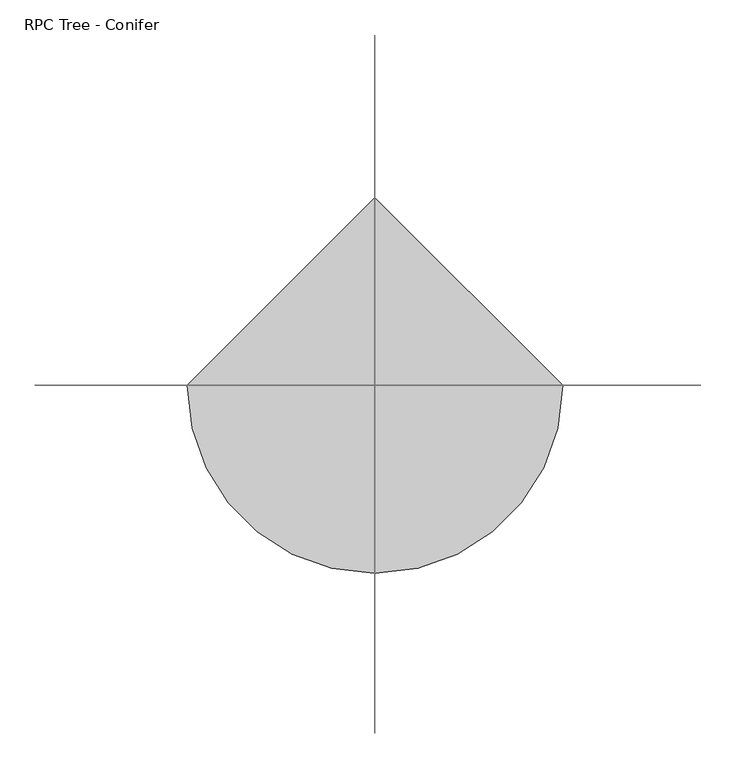
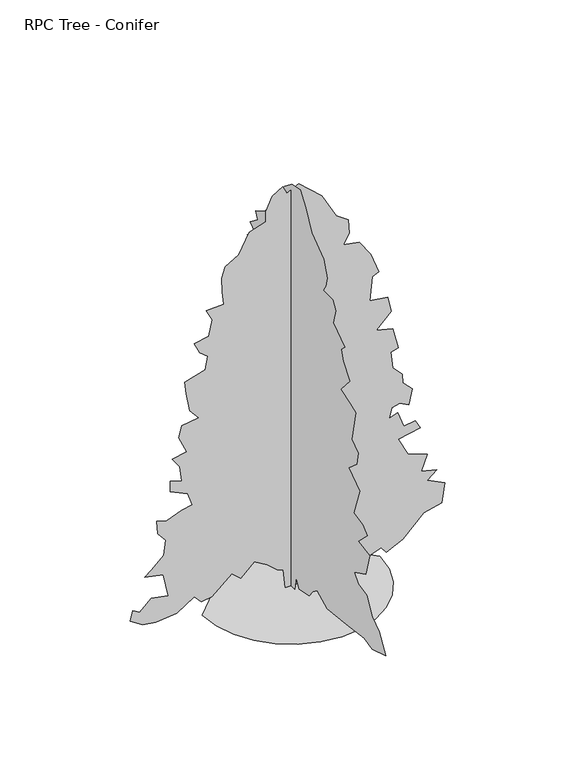
"""IFC4 building model written with IfcOpenShell, lengths in millimetres: geographic element geometry, RPC Tree - Conifer : Colorado Spruce - 4.0 Meters."""

from ifc_helpers import new_model, si_unit, origin, place, context, project, spatial, triangles, source, transform, mapped, element, save


def rpc_tree_conifer_283005fb(model_context):
    return source(origin(), model_context, "Body", "Tessellation", [
        triangles([(0.1966733, 49.8244978, 3.62e-05), (0.1966808, 76.8972503, 209.8139919), (0.1966851, 110.7382534, 304.5674924), (0.1966885, 232.565492, 236.886758), (0.1966934, 381.4650152, 175.9729979), (0.1967001, 550.6699851, 148.90025), (0.1967079, 720.3449844, 156.1022449), (0.1967054, 740.1799656, 40.6092491), (0.1967132, 862.0074858, 121.827502), (0.1967165, 991.2750315, 36.3350005), (0.1967216, 1085.3575155, 67.6820016), (0.1967296, 1268.1000675, 60.913751), (0.1967359, 1356.0849586, 142.1320039), (0.1967499, 1545.5950481, 324.872503), (0.1967463, 1430.5350655, 379.0174902), (0.1967428, 1329.0124832, 412.8600102), (0.1967383, 1234.4449997, 404.9599837), (0.1967407, 1213.9525005, 514.3824835), (0.1967447, 1241.024976, 609.1374919), (0.1967522, 1335.779948, 717.4275026), (0.1967485, 1241.024976, 737.7325132), (0.1967539, 1315.4749374, 805.4150099), (0.1967498, 1200.4174982, 839.2550228), (0.1967461, 1078.589978, 900.169982), (0.1967471, 1015.9549931, 1025.5049915), (0.1967554, 1173.3450228, 1069.3749882), (0.1967602, 1241.024976, 1130.2874765), (0.1967569, 1153.0400122, 1150.5924871), (0.1967529, 1004.1400166, 1238.5800671), (0.1967593, 1112.429991, 1292.7250179), (0.196765, 1121.189994, 1470.9574528), (0.19676, 997.3700083, 1489.0025723), (0.196756, 889.0800339, 1516.0750477), (0.1967604, 905.0550035, 1639.3949913), (0.1967674, 1036.9399767, 1676.5725185), (0.1967726, 1065.0525049, 1807.1074287), (0.1967671, 956.7625305, 1786.8025635), (0.196768, 888.3749897, 1918.5275173), (0.1967741, 963.5299953, 2010.1524479), (0.1967722, 868.7750233, 2091.3700195), (0.1967785, 963.5299953, 2159.0525162), (0.1967813, 990.6024708, 2213.197467), (0.196777, 821.3974646, 2321.4899849), (0.1967781, 801.0925266, 2389.1700108), (0.1967862, 936.4575199, 2456.8523621), (0.1967861, 875.5424881, 2544.8498978), (0.1967818, 740.1799656, 2605.7499596), (0.1967888, 828.1650021, 2707.2748672), (0.1967872, 733.41003, 2795.2500206), (0.1967844, 611.5849806, 2883.2498817), (0.1967873, 604.8150086, 2991.5499573), (0.1967932, 706.3374819, 3038.9249725), (0.1967915, 631.8899912, 3093.074865), (0.1967882, 543.9024839, 3113.3750793), (0.1967957, 658.9624666, 3194.5750648), (0.1967931, 537.1349828, 3289.3500938), (0.1967966, 570.9749957, 3357.0250328), (0.1967927, 428.8425013, 3438.2500168), (0.1967912, 313.7824822, 3560.0751389), (0.1967925, 237.8634971, 3716.3499023), (0.1967912, 97.2017522, 3884.9500763), (0.196789, -11.0894496, 3972.924939), (0.1967837, -146.4532518, 4000.0000305), (0.1967759, -241.2080059, 3878.1749084), (0.196766, -335.9624874, 3688.6751381), (0.196753, -532.2400054, 3546.5250938), (0.1967459, -586.3849926, 3390.8750015), (0.1967443, -559.3125172, 3296.0999725), (0.196744, -525.4725042, 3235.1999107), (0.1967374, -674.3724998, 3235.1999107), (0.1967328, -721.7499859, 3153.9749268), (0.1967304, -681.1399647, 3011.849881), (0.1967181, -870.6499815, 2883.2498817), (0.1967192, -809.7350224, 2829.0999893), (0.1967147, -843.5775061, 2727.5750816), (0.196706, -951.8674805, 2598.9750824), (0.1967076, -802.9674849, 2429.780032), (0.1966991, -959.7425085, 2380.804969), (0.1966941, -1046.6225252, 2341.7949955), (0.1966879, -985.7074934, 2043.9925335), (0.1966812, -1087.2324738, 1969.542572), (0.1966785, -1066.9275358, 1847.7149792), (0.1966808, -938.3300074, 1732.6574673), (0.1966693, -1114.3050219, 1610.8300198), (0.1966655, -1012.7825123, 1333.3325684), (0.1966581, -1161.6825079, 1306.2599476), (0.1966529, -1236.132542, 1245.3475319), (0.1966552, -1087.2324738, 1096.4475363), (0.1966459, -1276.7399471, 1069.3749882), (0.1966422, -1209.0599939, 846.0224876), (0.1966478, -1026.3175146, 758.0375238), (0.1966426, -1087.2324738, 676.8200249), (0.1966355, -1229.3624611, 649.7474768), (0.1966269, -1317.3499683, 494.0775092), (0.1966194, -1432.409951, 412.8600102), (0.1966096, -1533.9325333, 236.886758), (0.1966172, -1317.3499683, 169.2047519), (0.1966241, -1184.517524, 199.5652534), (0.1966359, -895.4949766, 164.0745054), (0.1966487, -586.3849926, 128.5955028), (0.1966584, -423.9474875, 209.8139919), (0.1966598, -356.267498, 155.6682416), (0.1966603, -295.3525025, 81.2182529), (0.1966665, -132.9167506, 47.3774997), (0.1966712, -85.8942484, 133.3167535), (0.1966685, -58.4667483, 3.3e-05), (-51.204578, 1.3e-06, 3.62e-05), (-71.5090799, -2.08e-05, 182.7412439), (-125.6545758, -2.01e-05, 203.0457458), (-220.4093299, -2.09e-05, 284.2650071), (-342.2358327, -2.06e-05, 358.7149867), (-470.8333248, 3.2e-06, 236.886758), (-552.0508238, 2.3e-06, 311.3375007), (-741.5608406, 1.52e-05, 148.90025), (-836.7233459, 1.86e-05, 136.9905027), (-903.9958385, 1.73e-05, 209.8139919), (-1066.4333799, 2.7e-05, 101.5230001), (-1262.7108616, 4.83e-05, 81.2184982), (-1384.5383091, 5.1e-05, 101.5230001), (-1499.5982918, 5.11e-05, 175.9729979), (-1479.2934265, 4.63e-05, 270.7274976), (-1411.6107845, 4.61e-05, 230.1184938), (-1303.318412, 2.38e-05, 331.6425113), (-1147.6508789, 2.04e-05, 304.5674924), (-1193.5583239, 1.17e-05, 528.1124957), (-1364.2332985, 1.53e-05, 561.7600059), (-1303.318412, 1.14e-05, 609.1374919), (-1188.2608274, 3.1e-06, 717.4275026), (-1167.9558895, -3.8e-06, 859.5600334), (-1242.405851, -5.5e-06, 947.547468), (-1255.9433968, -1.09e-05, 1076.1425257), (-1161.188352, -1.25e-05, 1049.0699776), (-1019.0558212, -3.37e-05, 1103.2150011), (-924.3008492, -3.74e-05, 1123.5200117), (-964.9108704, -4.17e-05, 1245.3475319), (-1127.4908449, -4.02e-05, 1321.492448), (-1127.3458683, -4.5e-05, 1428.0875404), (-1019.0558212, -4.67e-05, 1394.2474548), (-1037.3183693, -5.26e-05, 1538.1075691), (-1107.0433285, -5.5e-05, 1637.9024952), (-971.6783352, -6.02e-05, 1664.9749706), (-1046.1283693, -6.53e-05, 1827.4099686), (-1019.0558212, -7.09e-05, 1935.7024864), (-863.3883608, -9.13e-05, 1962.7749619), (-944.6058598, -9.31e-05, 2057.5299339), (-978.4458727, -0.0001002, 2240.2699425), (-991.9833458, -0.000105, 2355.3300705), (-802.473329, -0.0001134, 2416.2424862), (-775.4008535, -0.0001196, 2538.0750206), (-849.8508877, -0.0001201, 2598.9750824), (-903.9958385, -0.0001233, 2707.2748672), (-766.3633238, -0.000143, 2730.4499062), (-734.7908323, -0.0001508, 2883.2498817), (-788.9358559, -0.000154, 2991.5499573), (-626.5008579, -0.0001591, 2998.3001266), (-640.0358603, -0.0001645, 3126.9001259), (-646.8058685, -0.0001703, 3262.2750023), (-612.9633848, -0.0001759, 3363.79991), (-487.5108315, -0.0001976, 3440.9251442), (-389.6133187, -0.0002089, 3627.7500778), (-233.9455858, -0.0002156, 3675.1250931), (-233.9455858, -0.0002202, 3776.6500008), (-173.0318439, -0.0002277, 3905.25), (-78.277326, -0.0002333, 3966.1500618), (-37.6680791, -0.0002312, 3891.699955), (70.622924, -0.0002513, 3945.8501381), (287.2041627, -0.000249, 3749.5749092), (422.5691923, -0.0002276, 3505.9249557), (537.629175, -0.0002419, 3424.6999718), (544.3966762, -0.0002216, 3289.3500938), (490.251689, -0.0002157, 3194.5750648), (639.1516119, -0.000219, 3167.5249718), (747.441659, -0.0002152, 3011.849881), (821.8916204, -0.0002087, 2815.5749428), (760.3216141, -0.0002054, 2783.5498627), (733.9066566, -0.0001945, 2558.3749443), (903.1091194, -0.0001984, 2531.3001434), (936.9516758, -0.0001927, 2382.4025459), (794.819145, -0.0001824, 2247.0400234), (950.4866781, -0.0001853, 2206.4300022), (1004.6341724, -0.000163, 1996.6150475), (930.1816675, -0.0001602, 1983.0799725), (950.4866781, -0.0001535, 1820.6425037), (1039.9941507, -0.0001518, 1722.8699833), (1045.2416502, -0.0001482, 1637.9024952), (1133.2291574, -0.0001468, 1549.9149879), (1099.3866737, -0.0001392, 1401.015065), (1018.1691748, -0.0001389, 1448.392551), (943.7191406, -0.0001358, 1428.0875404), (916.6466652, -0.0001307, 1333.3325684), (997.8641642, -0.0001343, 1360.4050438), (1052.009115, -0.000129, 1204.7375107), (1160.3016329, -0.0001331, 1225.0425213), (1207.6791189, -0.0001306, 1137.055014), (1004.6341724, -0.0001227, 1096.4475363), (1092.6191362, -0.000103, 920.4725218), (1275.3616882, -0.0001199, 852.7924959), (1216.884153, -9.7e-05, 703.8949711), (1363.3465794, -9.98e-05, 670.0500166), (1275.3616882, -9.39e-05, 595.5999825), (1437.7966862, -9.51e-05, 514.3824835), (1410.7242107, -8.58e-05, 324.872503), (1241.5191319, -7.9e-05, 284.2650071), (1046.1716806, -6.47e-05, 94.2452466), (889.5741171, -4.22e-05, 20.3044996), (842.1966311, -4.35e-05, 81.2182529), (664.5366177, -3.55e-05, 20.9521254), (476.7141795, -2.96e-05, 13.5363501), (402.2641817, -3.04e-05, 81.2182529), (233.0594117, -2.8e-05, 142.1320039), (73.3656708, -2.18e-05, 109.4187482), (57.0864228, -1.64e-05, 3.3e-05), (-828.2308411, -4.6e-06, 5.94e-05), (-806.3283262, -189.8204993, 5.31e-05), (-743.9558252, -364.1399826, 4.6e-05), (-646.1033678, -517.9650046, 3.85e-05), (-517.7683233, -646.3000128, 3.09e-05), (-363.9433013, -744.1524702, 2.34e-05), (-189.6238362, -806.5249712, 1.63e-05), (0.1967073, -828.427486, 1e-05), (190.0171625, -806.5249712, 5e-06), (364.3366639, -744.1524702, 1.7e-06), (518.1616859, -646.3000128, 0.0), (646.4966578, -517.9650046, 0.0), (744.3491152, -364.1399826, 1.7e-06), (806.7216162, -189.8204993, 5e-06), (828.624131, 7.68e-05, 1e-05), (0.1965624, 828.427486, 5.94e-05)], [[26, 27, 28], [21, 22, 23], [19, 20, 21], [51, 52, 53], [7, 8, 9], [35, 36, 37], [13, 14, 15], [34, 35, 37], [54, 55, 56], [72, 73, 74], [95, 96, 97], [88, 89, 90], [44, 45, 46], [86, 87, 88], [85, 86, 88], [51, 53, 54], [44, 46, 47], [88, 90, 91], [13, 15, 16], [13, 16, 17], [38, 39, 40], [25, 26, 28], [25, 28, 29], [47, 48, 49], [56, 57, 58], [30, 31, 32], [29, 30, 32], [41, 42, 43], [40, 41, 43], [106, 1, 2], [105, 106, 2], [75, 76, 77], [94, 95, 97], [94, 97, 98], [78, 79, 80], [83, 84, 85], [29, 32, 33], [103, 104, 105], [12, 13, 17], [11, 12, 17], [77, 78, 80], [102, 103, 105], [62, 63, 64], [80, 81, 82], [80, 82, 83], [61, 62, 64], [61, 64, 65], [60, 61, 65], [59, 60, 65], [69, 70, 71], [69, 71, 72], [94, 98, 99], [93, 94, 99], [92, 93, 99], [92, 99, 100], [91, 92, 100], [91, 100, 101], [47, 49, 50], [9, 10, 11], [9, 11, 17], [9, 17, 18], [7, 9, 18], [59, 65, 66], [59, 66, 67], [59, 67, 68], [59, 68, 69], [58, 59, 69], [56, 58, 69], [54, 56, 69], [54, 69, 72], [51, 54, 72], [50, 51, 72], [50, 72, 74], [50, 74, 75], [50, 75, 77], [47, 50, 77], [44, 47, 77], [43, 44, 77], [40, 43, 77], [40, 77, 80], [40, 80, 83], [38, 40, 83], [38, 83, 85], [37, 38, 85], [34, 37, 85], [33, 34, 85], [29, 33, 85], [25, 29, 85], [25, 85, 88], [25, 88, 91], [25, 91, 101], [25, 101, 102], [24, 25, 102], [23, 24, 102], [21, 23, 102], [105, 2, 3], [102, 105, 3], [21, 102, 3], [21, 3, 4], [21, 4, 5], [21, 5, 6], [21, 6, 7], [21, 7, 18], [19, 21, 18], [125, 126, 127], [198, 199, 200], [153, 154, 155], [139, 140, 141], [130, 131, 132], [120, 121, 122], [119, 120, 122], [186, 187, 188], [136, 137, 138], [135, 136, 138], [150, 151, 152], [193, 194, 195], [192, 193, 195], [125, 127, 128], [180, 181, 182], [163, 164, 165], [185, 186, 188], [196, 197, 198], [190, 191, 192], [111, 112, 113], [212, 107, 108], [211, 212, 108], [173, 174, 175], [149, 150, 152], [179, 180, 182], [129, 130, 132], [146, 147, 148], [204, 205, 206], [200, 201, 202], [200, 202, 203], [162, 163, 165], [190, 192, 195], [165, 166, 167], [118, 119, 122], [118, 122, 123], [118, 123, 124], [117, 118, 124], [116, 117, 124], [176, 177, 178], [176, 178, 179], [129, 132, 133], [185, 188, 189], [142, 143, 144], [141, 142, 144], [161, 162, 165], [161, 165, 167], [161, 167, 168], [116, 124, 125], [145, 146, 148], [144, 145, 148], [114, 115, 116], [113, 114, 116], [113, 116, 125], [113, 125, 128], [113, 128, 129], [113, 129, 133], [113, 133, 134], [111, 113, 134], [168, 169, 170], [168, 170, 171], [161, 168, 171], [160, 161, 171], [159, 160, 171], [158, 159, 171], [157, 158, 171], [156, 157, 171], [155, 156, 171], [171, 172, 173], [171, 173, 175], [155, 171, 175], [155, 175, 176], [153, 155, 176], [152, 153, 176], [149, 152, 176], [149, 176, 179], [148, 149, 179], [144, 148, 179], [144, 179, 182], [144, 182, 183], [141, 144, 183], [139, 141, 183], [138, 139, 183], [135, 138, 183], [134, 135, 183], [111, 134, 183], [110, 111, 183], [110, 183, 184], [110, 184, 185], [110, 185, 189], [110, 189, 190], [110, 190, 195], [109, 110, 195], [108, 109, 195], [211, 108, 195], [210, 211, 195], [210, 195, 196], [209, 210, 196], [209, 196, 198], [208, 209, 198], [207, 208, 198], [206, 207, 198], [204, 206, 198], [203, 204, 198], [200, 203, 198], [227, 228, 213], [226, 227, 213], [226, 213, 214], [225, 226, 214], [225, 214, 215], [225, 215, 216], [224, 225, 216], [223, 224, 216], [223, 216, 217], [223, 217, 218], [223, 218, 219], [223, 219, 220], [223, 220, 221], [223, 221, 222]], closed=False),
    ])


if __name__ == "__main__":
    model = new_model("IFC4")
    model_context = context("Model", 3, world=origin())
    ifc_project = project(units=[si_unit("LENGTHUNIT", "METRE", prefix="MILLI")], contexts=[model_context])
    site = spatial("IfcSite", under=ifc_project)
    building = spatial("IfcBuilding", under=site)
    placement = place(None, origin())
    rpc_tree_conifer_shape = rpc_tree_conifer_283005fb(model_context)
    element("IfcGeographicElement", 1, ObjectType="RPC Tree - Conifer : Colorado Spruce - 4.0 Meters", at=placement, inside=building, context=model_context, shape_type="MappedRepresentation", body=[
        mapped(rpc_tree_conifer_shape, transform((0.0, 0.0, 0.0), x_axis=(1.0, 0.0, 0.0), y_axis=(0.0, 1.0, 0.0), z_axis=(0.0, 0.0, 1.0))),
    ])
    save(model, "model.ifc")

# Revit data of these elements
# Type "RPC Tree - Conifer : Colorado Spruce - 4.0 Meters"
#   built-in parameter 1005198 = "{2, 15},{39, RPC-16-G0M4-N9PX-U6TN-C000-ST1L-LVER-AU},{1, 0},{1, 0},{2, 13},{1, 8},{5, Color},{1, 0},{1, 0},{3, 0.8},{3, 0.8},{3, 0.8},{1, 8},{7, BBoxMin},{1, 0},{1, 0},{1, 0},{1, 0},{1, 0},{1, 8},{7, BBoxMax},{1, 0},{1, 0},{1, 0},{1, 0},{1, 0},{2, 11},{9, RPCTypeId},{1, 0},{1, 0},{39, RPC-16-G0M4-N9PX-U6TN-C000-ST1L-LVER-AU},{1, 6},{14, RPCPlantHeight},{1, 0},{1, 0},{7, 13.1234},{2, 11},{7, keyword},{1, 0},{1, 0},{34, :RPCs:Trees [General]:Geometry:RPC},{2, 11},{8, category},{1, 0},{1, 0},{15, Trees [General]},{2, 11},{12, LocalizedUID},{1, 0},{1, 0},{15, Colorado Spruce},{2, 14},{6, Height},{1, 0},{1, 0},{7, 13.1234},{1, 2},{16, Cast Reflections},{1, 0},{1, 0},{1, 0},{1, 2},{12, Cast Shadows},{1, 0},{1, 0},{1, 1},{1, 2},{9, Lock View},{1, 0},{1, 0},{1, 0},{1, 4},{5, ViewC},{1, 0},{1, 0},{1, 0},{21, assetlibrary_base.fbx},{1, 5},"
#   built-in parameter 1005195 = "RPC-16-G0M4-N9PX-U6TN-C000-ST1L-LVER-AU"
#   Type Comments = "Colorado Spruce"
#   Height = 4000 mm
#   Description = (empty or 0)
#   Default Elevation = 0
